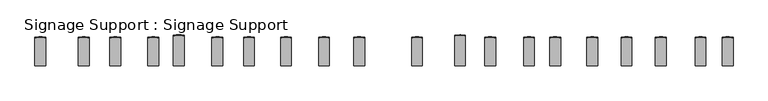
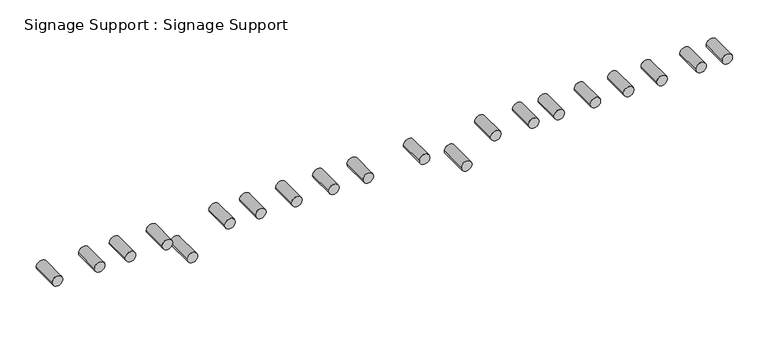
"""IFC4 building model written with IfcOpenShell, lengths in millimetres: proxy geometry, Signage Support : Signage Support."""

import ifcopenshell
import ifcopenshell.guid

model = None  # the IFC model being written
_history = None  # IfcOwnerHistory: only IFC2X3 demands one
_inside = {}  # id of a spatial element -> (the spatial element, [elements in it])
_under = {}  # id of a project, library or spatial element -> (it, [spatial elements below it])
_declared = {}  # id of a project -> (the project, [libraries it declares])
_typed = {}  # id of a type object -> (the type object, [elements of that type])
_made_of = {}  # id of a material, layer set ... -> (it, [elements and type objects made of it])


def new_model(schema):
    """Start an empty IFC model of exactly this schema.

    Asked for "IFC4X3", IfcOpenShell would pick the latest addendum, in which some entities
    have other attributes; the version numbers below select the first issue.
    IFC2X3 requires an IfcOwnerHistory on every rooted entity: one is made here for all.
    """
    global model, _history
    if schema == "IFC4X3":
        model = ifcopenshell.file(schema_version=(4, 3, 0, 0))
    else:
        model = ifcopenshell.file(schema=schema)
    _inside.clear()
    _under.clear()
    _declared.clear()
    _typed.clear()
    _made_of.clear()
    _history = None
    if model.schema == "IFC2X3":
        org = make("IfcOrganization", Name="unknown")
        user = make(
            "IfcPersonAndOrganization",
            ThePerson=make("IfcPerson", FamilyName="unknown"),
            TheOrganization=org,
        )
        app = make(
            "IfcApplication",
            ApplicationDeveloper=org,
            Version="unknown",
            ApplicationFullName="unknown",
            ApplicationIdentifier="unknown",
        )
        _history = make(
            "IfcOwnerHistory",
            OwningUser=user,
            OwningApplication=app,
            ChangeAction="ADDED",
            CreationDate=0,
        )
    return model


def make(cls, **values):
    """One entity of the class cls with the attributes given. An attribute that is None is left unset."""
    return model.create_entity(
        cls, **{name: value for name, value in values.items() if value is not None}
    )


def rooted(cls, **values):
    """An entity with a GlobalId (a new one), such as an element, a storey or a relation."""
    return make(cls, GlobalId=ifcopenshell.guid.new(), OwnerHistory=_history, **values)


def si_unit(unit_type, name, prefix=None):
    """IfcSIUnit, for example si_unit("LENGTHUNIT", "METRE", prefix="MILLI")."""
    return make("IfcSIUnit", UnitType=unit_type, Prefix=prefix, Name=name)


def assignment(units):
    """IfcUnitAssignment: the units of a project."""
    return None if units is None else make("IfcUnitAssignment", Units=units)


def point(xyz):
    """IfcCartesianPoint."""
    return None if xyz is None else make("IfcCartesianPoint", Coordinates=xyz)


def direction(xyz):
    """IfcDirection."""
    return None if xyz is None else make("IfcDirection", DirectionRatios=xyz)


def frame(location, z_axis=None, x_axis=None):
    """IfcAxis2Placement3D, a coordinate frame: its origin and axes. An axis left out is left unset."""
    return make(
        "IfcAxis2Placement3D",
        Location=point(location),
        Axis=direction(z_axis),
        RefDirection=direction(x_axis),
    )


def origin():
    """The frame at (0, 0, 0) with its axes left unset."""
    return frame((0.0, 0.0, 0.0))


def place(relative_to, where):
    """IfcLocalPlacement: puts the frame where relative to a parent placement (None: the world)."""
    return make(
        "IfcLocalPlacement", PlacementRelTo=relative_to, RelativePlacement=where
    )


def context(
    kind, dimensions, precision=None, world=None, true_north=None, identifier=None
):
    """IfcGeometricRepresentationContext, for example the 3D "Model" context."""
    return make(
        "IfcGeometricRepresentationContext",
        ContextIdentifier=identifier,
        ContextType=kind,
        CoordinateSpaceDimension=dimensions,
        Precision=precision,
        WorldCoordinateSystem=world,
        TrueNorth=true_north,
    )


def project(units=None, contexts=None):
    """IfcProject with its units and contexts."""
    return rooted(
        "IfcProject",
        Name="project",
        RepresentationContexts=contexts,
        UnitsInContext=assignment(units),
    )


def spatial(cls, under=None, at=None, **own):
    """A site, building, storey or space (cls), placed at a placement, below another one or the project."""
    s = rooted(cls, ObjectPlacement=at, **own)
    if under is not None:
        _under.setdefault(under.id(), (under, []))[1].append(s)
    return s


def circle_curve(where, radius):
    """IfcCircle in the frame where."""
    return make("IfcCircle", Position=where, Radius=radius)


def ellipse_curve(where, semi_axis1, semi_axis2):
    """IfcEllipse in the frame where."""
    return make(
        "IfcEllipse", Position=where, SemiAxis1=semi_axis1, SemiAxis2=semi_axis2
    )


def shape(context_of_items, identifier, shape_type, items):
    """IfcShapeRepresentation: the items that make up one representation, for example the "Body"."""
    return make(
        "IfcShapeRepresentation",
        ContextOfItems=context_of_items,
        RepresentationIdentifier=identifier,
        RepresentationType=shape_type,
        Items=items,
    )


def source(mapping_origin, context_of_items, identifier, shape_type, items):
    """IfcRepresentationMap: a shape defined once, which mapped items show again and again."""
    return make(
        "IfcRepresentationMap",
        MappingOrigin=mapping_origin,
        MappedRepresentation=shape(context_of_items, identifier, shape_type, items),
    )


def transform(
    local_origin,
    x_axis=None,
    y_axis=None,
    z_axis=None,
    scale=None,
    scale2=None,
    scale3=None,
    uniform=True,
):
    """IfcCartesianTransformationOperator3D, or its non-uniform kind. x_axis, y_axis, z_axis: its Axis1, 2, 3."""
    if uniform:
        return make(
            "IfcCartesianTransformationOperator3D",
            Axis1=direction(x_axis),
            Axis2=direction(y_axis),
            LocalOrigin=point(local_origin),
            Scale=scale,
            Axis3=direction(z_axis),
        )
    return make(
        "IfcCartesianTransformationOperator3DnonUniform",
        Axis1=direction(x_axis),
        Axis2=direction(y_axis),
        LocalOrigin=point(local_origin),
        Scale=scale,
        Axis3=direction(z_axis),
        Scale2=scale2,
        Scale3=scale3,
    )


def mapped(mapping_source, mapping_target):
    """IfcMappedItem: shows the shape of a source again, moved by a transform."""
    return make(
        "IfcMappedItem", MappingSource=mapping_source, MappingTarget=mapping_target
    )


def made_of(thing, what):
    """Note that an element or type object is made of a material, layer set ...; save() writes the relation."""
    if what is not None:
        _made_of.setdefault(what.id(), (what, []))[1].append(thing)
    return thing


def element(
    cls,
    number,
    at=None,
    inside=None,
    cuts=None,
    type_object=None,
    material=None,
    context=None,
    identifier="Body",
    shape_type=None,
    held_by="IfcProductDefinitionShape",
    body=None,
    shapes=None,
    **own,
):
    """One element of the class cls, such as IfcWall. Its Tag is "e" and its number.

    at: its placement. inside: the storey or other place that contains it. cuts: it is an
    opening in that element (IfcRelVoidsElement). A single representation is given by context,
    identifier, shape_type and body (its items); several are given by shapes. held_by: the class
    of the entity that holds the representations. save() writes the other relations.
    """
    e = rooted(cls, Tag="e%d" % number, ObjectPlacement=at, **own)
    if body is not None:
        shapes = [shape(context, identifier, shape_type, body)]
    if shapes is not None:
        e.Representation = make(held_by, Representations=shapes)
    if inside is not None:
        _inside.setdefault(inside.id(), (inside, []))[1].append(e)
    if cuts is not None:
        rooted(
            "IfcRelVoidsElement", RelatingBuildingElement=cuts, RelatedOpeningElement=e
        )
    if type_object is not None:
        _typed.setdefault(type_object.id(), (type_object, []))[1].append(e)
    return made_of(e, material)


def aggregate(whole, parts):
    """IfcRelAggregates: a whole, such as a stair, and the parts it consists of."""
    return rooted("IfcRelAggregates", RelatingObject=whole, RelatedObjects=parts)


def save(model, path):
    """Write the relations noted so far, then the file.

    IfcRelAggregates (storeys below a building ...), IfcRelContainedInSpatialStructure (elements
    in a storey), IfcRelDefinesByType, IfcRelAssociatesMaterial and IfcRelDeclares: one each for
    every whole, place, type object, material and project.
    """
    for whole, parts in _under.values():
        aggregate(whole, parts)
    for where, things in _inside.values():
        rooted(
            "IfcRelContainedInSpatialStructure",
            RelatedElements=things,
            RelatingStructure=where,
        )
    for kind, things in _typed.values():
        rooted("IfcRelDefinesByType", RelatedObjects=things, RelatingType=kind)
    for what, things in _made_of.values():
        rooted("IfcRelAssociatesMaterial", RelatedObjects=things, RelatingMaterial=what)
    for by, libraries in _declared.values():
        rooted("IfcRelDeclares", RelatingContext=by, RelatedDefinitions=libraries)
    model.write(path)


def plane_surface(at):
    """IfcPlane: the flat surface through the origin of the frame at, square to its z axis."""
    return make("IfcPlane", Position=at)


def cylinder_surface(at, radius):
    """IfcCylindricalSurface: all points at the distance radius from the z axis of the frame at."""
    return make("IfcCylindricalSurface", Position=at, Radius=radius)


def advanced_brep(points, edges, surfaces, faces):
    """IfcAdvancedBrep: a solid bounded by faces that lie on surfaces and meet in shared edges.

    An edge is (start, end): straight between two places in points (the first is 0);
    or (start, end, curve); or (start, end, curve, False) where it runs against its curve.
    A face is (place in surfaces, loops), or (place, loops, False) where it looks against
    its surface's normal. A loop lists edges by number (the first is 1), with a minus sign
    where the edge is run from its end to its start. The first loop is the outer one.
    """
    corners = [point(p) for p in points]
    vertices = [make("IfcVertexPoint", VertexGeometry=c) for c in corners]
    made = []
    for start, end, *more in edges:
        made.append(
            make(
                "IfcEdgeCurve",
                EdgeStart=vertices[start],
                EdgeEnd=vertices[end],
                EdgeGeometry=more[0] if more else make("IfcPolyline", Points=[corners[start], corners[end]]),
                SameSense=more[1] if len(more) > 1 else True,
            )
        )
    hull = []
    for where, loops, *sense in faces:
        bounds = []
        for j, loop in enumerate(loops):
            ring = [make("IfcOrientedEdge", EdgeElement=made[abs(k) - 1], Orientation=k > 0) for k in loop]
            bounds.append(
                make(
                    "IfcFaceOuterBound" if j == 0 else "IfcFaceBound",
                    Bound=make("IfcEdgeLoop", EdgeList=ring),
                    Orientation=True,
                )
            )
        hull.append(make("IfcAdvancedFace", Bounds=bounds, FaceSurface=surfaces[where], SameSense=sense[0] if sense else True))
    return make("IfcAdvancedBrep", Outer=make("IfcClosedShell", CfsFaces=hull))


def signage_support_signage_support_2350426c(model_context):
    return source(origin(), model_context, "Body", "AdvancedBrep", [
        advanced_brep(
        [(16177.267357, -19458.5804995, 34584.5182697), (16253.467357, -19458.5804995, 34584.5182697), (16253.467357, -19245.9211169, 34584.5182697), (16177.267357, -19245.9211169, 34584.5182697)],
        [
            (0, 1, circle_curve(frame((16215.367357, -19458.5804995, 34584.5182697), z_axis=(0.0, -1.0, 0.0), x_axis=(1.0, 0.0, 0.0)), 38.1)),
            (1, 0, circle_curve(frame((16215.367357, -19458.5804995, 34584.5182697), z_axis=(0.0, -1.0, 0.0), x_axis=(1.0, 0.0, 0.0)), 38.1)),
            (1, 2),
            (2, 3, ellipse_curve(frame((16215.367357, -19245.9211169, 34584.5182697), z_axis=(0.0, -0.9961946980917453, -0.08715574274766139), x_axis=(0.0, 0.08715574274765964, -0.9961946980917453)), 38.2455358, 38.1)),
            (3, 0),
            (3, 2, ellipse_curve(frame((16215.367357, -19245.9211169, 34584.5182697), z_axis=(0.0, -0.9961946980917453, -0.08715574274766139), x_axis=(0.0, 0.08715574274765964, -0.9961946980917453)), 38.2455358, 38.1)),
        ],
        [
            plane_surface(frame((15807.4961456, -19458.5804995, 34748.2945741), z_axis=(0.0, -1.0, 0.0), x_axis=(0.0, 0.0, 1.0))),
            cylinder_surface(frame((16215.367357, -19458.5804995, 34584.5182697), z_axis=(0.0, 1.0, 0.0), x_axis=(1.0, 0.0, 0.0)), 38.1),
            plane_surface(frame((2527.7462086, -19227.8856773, 34378.3722523), z_axis=(0.0, 0.9961946980917453, 0.08715574274766139), x_axis=(1.0, 0.0, 0.0))),
        ],
        [
            (0, [[1, 2]]),
            (1, [[-2, 3, 4, 5]]),
            (1, [[-1, -5, 6, -3]]),
            (2, [[-4, -6]]),
        ],
    ),
        advanced_brep(
        [(15731.2961456, -19458.5804995, 34748.2945741), (15807.4961456, -19458.5804995, 34748.2945741), (15807.4961456, -19260.2496869, 34748.2945741), (15731.2961456, -19260.2496869, 34748.2945741)],
        [
            (0, 1, circle_curve(frame((15769.3961456, -19458.5804995, 34748.2945741), z_axis=(0.0, 1.0, 0.0), x_axis=(1.0, 0.0, 0.0)), 38.1)),
            (1, 2),
            (2, 3, ellipse_curve(frame((15769.3961456, -19260.2496869, 34748.2945741), z_axis=(0.0, -0.9961946980917453, -0.08715574274766139), x_axis=(0.0, 0.08715574274765964, -0.9961946980917453)), 38.2455358, 38.1)),
            (3, 0),
            (1, 0, circle_curve(frame((15769.3961456, -19458.5804995, 34748.2945741), z_axis=(0.0, 1.0, 0.0), x_axis=(1.0, 0.0, 0.0)), 38.1)),
            (3, 2, ellipse_curve(frame((15769.3961456, -19260.2496869, 34748.2945741), z_axis=(0.0, -0.9961946980917453, -0.08715574274766139), x_axis=(0.0, 0.08715574274765964, -0.9961946980917453)), 38.2455358, 38.1)),
        ],
        [
            cylinder_surface(frame((15769.3961456, -19458.5804995, 34748.2945741), z_axis=(0.0, 1.0, 0.0), x_axis=(1.0, 0.0, 0.0)), 38.1),
            plane_surface(frame((15807.4961456, -19458.5804995, 34748.2945741), z_axis=(0.0, -1.0, 0.0), x_axis=(0.0, 0.0, 1.0))),
            plane_surface(frame((2527.7462086, -19227.8856773, 34378.3722523), z_axis=(0.0, 0.9961946980917453, 0.08715574274766139), x_axis=(1.0, 0.0, 0.0))),
        ],
        [
            (0, [[1, 2, 3, 4]]),
            (0, [[5, -4, 6, -2]]),
            (1, [[-5, -1]]),
            (2, [[-3, -6]]),
        ],
    ),
        advanced_brep(
        [(15997.9961456, -19458.5804995, 34748.2945741), (16074.1961456, -19458.5804995, 34748.2945741), (16074.1961456, -19260.2496869, 34748.2945741), (15997.9961456, -19260.2496869, 34748.2945741)],
        [
            (0, 1, circle_curve(frame((16036.0961456, -19458.5804995, 34748.2945741), z_axis=(0.0, 1.0, 0.0), x_axis=(1.0, 0.0, 0.0)), 38.1)),
            (1, 2),
            (2, 3, ellipse_curve(frame((16036.0961456, -19260.2496869, 34748.2945741), z_axis=(0.0, -0.9961946980917453, -0.08715574274766139), x_axis=(0.0, 0.08715574274765964, -0.9961946980917453)), 38.2455358, 38.1)),
            (3, 0),
            (1, 0, circle_curve(frame((16036.0961456, -19458.5804995, 34748.2945741), z_axis=(0.0, 1.0, 0.0), x_axis=(1.0, 0.0, 0.0)), 38.1)),
            (3, 2, ellipse_curve(frame((16036.0961456, -19260.2496869, 34748.2945741), z_axis=(0.0, -0.9961946980917453, -0.08715574274766139), x_axis=(0.0, 0.08715574274765964, -0.9961946980917453)), 38.2455358, 38.1)),
        ],
        [
            cylinder_surface(frame((16036.0961456, -19458.5804995, 34748.2945741), z_axis=(0.0, 1.0, 0.0), x_axis=(1.0, 0.0, 0.0)), 38.1),
            plane_surface(frame((15807.4961456, -19458.5804995, 34748.2945741), z_axis=(0.0, -1.0, 0.0), x_axis=(0.0, 0.0, 1.0))),
            plane_surface(frame((2527.7462086, -19227.8856773, 34378.3722523), z_axis=(0.0, 0.9961946980917453, 0.08715574274766139), x_axis=(1.0, 0.0, 0.0))),
        ],
        [
            (0, [[1, 2, 3, 4]]),
            (0, [[5, -4, 6, -2]]),
            (1, [[-5, -1]]),
            (2, [[-3, -6]]),
        ],
    ),
        advanced_brep(
        [(16448.8461456, -19458.5804995, 34748.2945741), (16525.0461456, -19458.5804995, 34748.2945741), (16525.0461456, -19260.2496869, 34748.2945741), (16448.8461456, -19260.2496869, 34748.2945741)],
        [
            (0, 1, circle_curve(frame((16486.9461456, -19458.5804995, 34748.2945741), z_axis=(0.0, 1.0, 0.0), x_axis=(1.0, 0.0, 0.0)), 38.1)),
            (1, 2),
            (2, 3, ellipse_curve(frame((16486.9461456, -19260.2496869, 34748.2945741), z_axis=(0.0, -0.9961946980917453, -0.08715574274766139), x_axis=(0.0, 0.08715574274765964, -0.9961946980917453)), 38.2455358, 38.1)),
            (3, 0),
            (1, 0, circle_curve(frame((16486.9461456, -19458.5804995, 34748.2945741), z_axis=(0.0, 1.0, 0.0), x_axis=(1.0, 0.0, 0.0)), 38.1)),
            (3, 2, ellipse_curve(frame((16486.9461456, -19260.2496869, 34748.2945741), z_axis=(0.0, -0.9961946980917453, -0.08715574274766139), x_axis=(0.0, 0.08715574274765964, -0.9961946980917453)), 38.2455358, 38.1)),
        ],
        [
            cylinder_surface(frame((16486.9461456, -19458.5804995, 34748.2945741), z_axis=(0.0, 1.0, 0.0), x_axis=(1.0, 0.0, 0.0)), 38.1),
            plane_surface(frame((15807.4961456, -19458.5804995, 34748.2945741), z_axis=(0.0, -1.0, 0.0), x_axis=(0.0, 0.0, 1.0))),
            plane_surface(frame((2527.7462086, -19227.8856773, 34378.3722523), z_axis=(0.0, 0.9961946980917453, 0.08715574274766139), x_axis=(1.0, 0.0, 0.0))),
        ],
        [
            (0, [[1, 2, 3, 4]]),
            (0, [[5, -4, 6, -2]]),
            (1, [[-5, -1]]),
            (2, [[-3, -6]]),
        ],
    ),
        advanced_brep(
        [(15509.0461456, -19458.5804995, 34748.2945741), (15585.2461456, -19458.5804995, 34748.2945741), (15585.2461456, -19260.2496869, 34748.2945741), (15509.0461456, -19260.2496869, 34748.2945741)],
        [
            (0, 1, circle_curve(frame((15547.1461456, -19458.5804995, 34748.2945741), z_axis=(0.0, 1.0, 0.0), x_axis=(1.0, 0.0, 0.0)), 38.1)),
            (1, 2),
            (2, 3, ellipse_curve(frame((15547.1461456, -19260.2496869, 34748.2945741), z_axis=(0.0, -0.9961946980917453, -0.08715574274766139), x_axis=(0.0, 0.08715574274765964, -0.9961946980917453)), 38.2455358, 38.1)),
            (3, 0),
            (1, 0, circle_curve(frame((15547.1461456, -19458.5804995, 34748.2945741), z_axis=(0.0, 1.0, 0.0), x_axis=(1.0, 0.0, 0.0)), 38.1)),
            (3, 2, ellipse_curve(frame((15547.1461456, -19260.2496869, 34748.2945741), z_axis=(0.0, -0.9961946980917453, -0.08715574274766139), x_axis=(0.0, 0.08715574274765964, -0.9961946980917453)), 38.2455358, 38.1)),
        ],
        [
            cylinder_surface(frame((15547.1461456, -19458.5804995, 34748.2945741), z_axis=(0.0, 1.0, 0.0), x_axis=(1.0, 0.0, 0.0)), 38.1),
            plane_surface(frame((15807.4961456, -19458.5804995, 34748.2945741), z_axis=(0.0, -1.0, 0.0), x_axis=(0.0, 0.0, 1.0))),
            plane_surface(frame((2527.7462086, -19227.8856773, 34378.3722523), z_axis=(0.0, 0.9961946980917453, 0.08715574274766139), x_axis=(1.0, 0.0, 0.0))),
        ],
        [
            (0, [[1, 2, 3, 4]]),
            (0, [[5, -4, 6, -2]]),
            (1, [[-5, -1]]),
            (2, [[-3, -6]]),
        ],
    ),
        advanced_brep(
        [(15204.2461456, -19458.5804995, 34748.2945741), (15280.4461456, -19458.5804995, 34748.2945741), (15280.4461456, -19260.2496869, 34748.2945741), (15204.2461456, -19260.2496869, 34748.2945741)],
        [
            (0, 1, circle_curve(frame((15242.3461456, -19458.5804995, 34748.2945741), z_axis=(0.0, 1.0, 0.0), x_axis=(1.0, 0.0, 0.0)), 38.1)),
            (1, 2),
            (2, 3, ellipse_curve(frame((15242.3461456, -19260.2496869, 34748.2945741), z_axis=(0.0, -0.9961946980917453, -0.08715574274766139), x_axis=(0.0, 0.08715574274765964, -0.9961946980917453)), 38.2455358, 38.1)),
            (3, 0),
            (1, 0, circle_curve(frame((15242.3461456, -19458.5804995, 34748.2945741), z_axis=(0.0, 1.0, 0.0), x_axis=(1.0, 0.0, 0.0)), 38.1)),
            (3, 2, ellipse_curve(frame((15242.3461456, -19260.2496869, 34748.2945741), z_axis=(0.0, -0.9961946980917453, -0.08715574274766139), x_axis=(0.0, 0.08715574274765964, -0.9961946980917453)), 38.2455358, 38.1)),
        ],
        [
            cylinder_surface(frame((15242.3461456, -19458.5804995, 34748.2945741), z_axis=(0.0, 1.0, 0.0), x_axis=(1.0, 0.0, 0.0)), 38.1),
            plane_surface(frame((15807.4961456, -19458.5804995, 34748.2945741), z_axis=(0.0, -1.0, 0.0), x_axis=(0.0, 0.0, 1.0))),
            plane_surface(frame((2527.7462086, -19227.8856773, 34378.3722523), z_axis=(0.0, 0.9961946980917453, 0.08715574274766139), x_axis=(1.0, 0.0, 0.0))),
        ],
        [
            (0, [[1, 2, 3, 4]]),
            (0, [[5, -4, 6, -2]]),
            (1, [[-5, -1]]),
            (2, [[-3, -6]]),
        ],
    ),
        advanced_brep(
        [(16671.0961456, -19458.5804995, 34748.2945741), (16747.2961456, -19458.5804995, 34748.2945741), (16747.2961456, -19260.2496869, 34748.2945741), (16671.0961456, -19260.2496869, 34748.2945741)],
        [
            (0, 1, circle_curve(frame((16709.1961456, -19458.5804995, 34748.2945741), z_axis=(0.0, 1.0, 0.0), x_axis=(1.0, 0.0, 0.0)), 38.1)),
            (1, 2),
            (2, 3, ellipse_curve(frame((16709.1961456, -19260.2496869, 34748.2945741), z_axis=(0.0, -0.9961946980917453, -0.08715574274766139), x_axis=(0.0, 0.08715574274765964, -0.9961946980917453)), 38.2455358, 38.1)),
            (3, 0),
            (1, 0, circle_curve(frame((16709.1961456, -19458.5804995, 34748.2945741), z_axis=(0.0, 1.0, 0.0), x_axis=(1.0, 0.0, 0.0)), 38.1)),
            (3, 2, ellipse_curve(frame((16709.1961456, -19260.2496869, 34748.2945741), z_axis=(0.0, -0.9961946980917453, -0.08715574274766139), x_axis=(0.0, 0.08715574274765964, -0.9961946980917453)), 38.2455358, 38.1)),
        ],
        [
            cylinder_surface(frame((16709.1961456, -19458.5804995, 34748.2945741), z_axis=(0.0, 1.0, 0.0), x_axis=(1.0, 0.0, 0.0)), 38.1),
            plane_surface(frame((15807.4961456, -19458.5804995, 34748.2945741), z_axis=(0.0, -1.0, 0.0), x_axis=(0.0, 0.0, 1.0))),
            plane_surface(frame((2527.7462086, -19227.8856773, 34378.3722523), z_axis=(0.0, 0.9961946980917453, 0.08715574274766139), x_axis=(1.0, 0.0, 0.0))),
        ],
        [
            (0, [[1, 2, 3, 4]]),
            (0, [[5, -4, 6, -2]]),
            (1, [[-5, -1]]),
            (2, [[-3, -6]]),
        ],
    ),
        advanced_brep(
        [(16931.4461456, -19458.5804995, 34748.2945741), (17007.6461456, -19458.5804995, 34748.2945741), (17007.6461456, -19260.2496869, 34748.2945741), (16931.4461456, -19260.2496869, 34748.2945741)],
        [
            (0, 1, circle_curve(frame((16969.5461456, -19458.5804995, 34748.2945741), z_axis=(0.0, 1.0, 0.0), x_axis=(1.0, 0.0, 0.0)), 38.1)),
            (1, 2),
            (2, 3, ellipse_curve(frame((16969.5461456, -19260.2496869, 34748.2945741), z_axis=(0.0, -0.9961946980917453, -0.08715574274766139), x_axis=(0.0, 0.08715574274765964, -0.9961946980917453)), 38.2455358, 38.1)),
            (3, 0),
            (1, 0, circle_curve(frame((16969.5461456, -19458.5804995, 34748.2945741), z_axis=(0.0, 1.0, 0.0), x_axis=(1.0, 0.0, 0.0)), 38.1)),
            (3, 2, ellipse_curve(frame((16969.5461456, -19260.2496869, 34748.2945741), z_axis=(0.0, -0.9961946980917453, -0.08715574274766139), x_axis=(0.0, 0.08715574274765964, -0.9961946980917453)), 38.2455358, 38.1)),
        ],
        [
            cylinder_surface(frame((16969.5461456, -19458.5804995, 34748.2945741), z_axis=(0.0, 1.0, 0.0), x_axis=(1.0, 0.0, 0.0)), 38.1),
            plane_surface(frame((15807.4961456, -19458.5804995, 34748.2945741), z_axis=(0.0, -1.0, 0.0), x_axis=(0.0, 0.0, 1.0))),
            plane_surface(frame((2527.7462086, -19227.8856773, 34378.3722523), z_axis=(0.0, 0.9961946980917453, 0.08715574274766139), x_axis=(1.0, 0.0, 0.0))),
        ],
        [
            (0, [[1, 2, 3, 4]]),
            (0, [[5, -4, 6, -2]]),
            (1, [[-5, -1]]),
            (2, [[-3, -6]]),
        ],
    ),
        advanced_brep(
        [(17198.1461456, -19458.5804995, 34748.2945741), (17274.3461456, -19458.5804995, 34748.2945741), (17274.3461456, -19260.2496869, 34748.2945741), (17198.1461456, -19260.2496869, 34748.2945741)],
        [
            (0, 1, circle_curve(frame((17236.2461456, -19458.5804995, 34748.2945741), z_axis=(0.0, 1.0, 0.0), x_axis=(1.0, 0.0, 0.0)), 38.1)),
            (1, 2),
            (2, 3, ellipse_curve(frame((17236.2461456, -19260.2496869, 34748.2945741), z_axis=(0.0, -0.9961946980917453, -0.08715574274766139), x_axis=(0.0, 0.08715574274765964, -0.9961946980917453)), 38.2455358, 38.1)),
            (3, 0),
            (1, 0, circle_curve(frame((17236.2461456, -19458.5804995, 34748.2945741), z_axis=(0.0, 1.0, 0.0), x_axis=(1.0, 0.0, 0.0)), 38.1)),
            (3, 2, ellipse_curve(frame((17236.2461456, -19260.2496869, 34748.2945741), z_axis=(0.0, -0.9961946980917453, -0.08715574274766139), x_axis=(0.0, 0.08715574274765964, -0.9961946980917453)), 38.2455358, 38.1)),
        ],
        [
            cylinder_surface(frame((17236.2461456, -19458.5804995, 34748.2945741), z_axis=(0.0, 1.0, 0.0), x_axis=(1.0, 0.0, 0.0)), 38.1),
            plane_surface(frame((15807.4961456, -19458.5804995, 34748.2945741), z_axis=(0.0, -1.0, 0.0), x_axis=(0.0, 0.0, 1.0))),
            plane_surface(frame((2527.7462086, -19227.8856773, 34378.3722523), z_axis=(0.0, 0.9961946980917453, 0.08715574274766139), x_axis=(1.0, 0.0, 0.0))),
        ],
        [
            (0, [[1, 2, 3, 4]]),
            (0, [[5, -4, 6, -2]]),
            (1, [[-5, -1]]),
            (2, [[-3, -6]]),
        ],
    ),
        advanced_brep(
        [(17445.7961456, -19458.5804995, 34748.2945741), (17521.9961456, -19458.5804995, 34748.2945741), (17521.9961456, -19260.2496869, 34748.2945741), (17445.7961456, -19260.2496869, 34748.2945741)],
        [
            (0, 1, circle_curve(frame((17483.8961456, -19458.5804995, 34748.2945741), z_axis=(0.0, 1.0, 0.0), x_axis=(1.0, 0.0, 0.0)), 38.1)),
            (1, 2),
            (2, 3, ellipse_curve(frame((17483.8961456, -19260.2496869, 34748.2945741), z_axis=(0.0, -0.9961946980917453, -0.08715574274766139), x_axis=(0.0, 0.08715574274765964, -0.9961946980917453)), 38.2455358, 38.1)),
            (3, 0),
            (1, 0, circle_curve(frame((17483.8961456, -19458.5804995, 34748.2945741), z_axis=(0.0, 1.0, 0.0), x_axis=(1.0, 0.0, 0.0)), 38.1)),
            (3, 2, ellipse_curve(frame((17483.8961456, -19260.2496869, 34748.2945741), z_axis=(0.0, -0.9961946980917453, -0.08715574274766139), x_axis=(0.0, 0.08715574274765964, -0.9961946980917453)), 38.2455358, 38.1)),
        ],
        [
            cylinder_surface(frame((17483.8961456, -19458.5804995, 34748.2945741), z_axis=(0.0, 1.0, 0.0), x_axis=(1.0, 0.0, 0.0)), 38.1),
            plane_surface(frame((15807.4961456, -19458.5804995, 34748.2945741), z_axis=(0.0, -1.0, 0.0), x_axis=(0.0, 0.0, 1.0))),
            plane_surface(frame((2527.7462086, -19227.8856773, 34378.3722523), z_axis=(0.0, 0.9961946980917453, 0.08715574274766139), x_axis=(1.0, 0.0, 0.0))),
        ],
        [
            (0, [[1, 2, 3, 4]]),
            (0, [[5, -4, 6, -2]]),
            (1, [[-5, -1]]),
            (2, [[-3, -6]]),
        ],
    ),
        advanced_brep(
        [(17852.1961456, -19458.5804995, 34748.2945741), (17928.3961456, -19458.5804995, 34748.2945741), (17928.3961456, -19260.2496869, 34748.2945741), (17852.1961456, -19260.2496869, 34748.2945741)],
        [
            (0, 1, circle_curve(frame((17890.2961456, -19458.5804995, 34748.2945741), z_axis=(0.0, 1.0, 0.0), x_axis=(1.0, 0.0, 0.0)), 38.1)),
            (1, 2),
            (2, 3, ellipse_curve(frame((17890.2961456, -19260.2496869, 34748.2945741), z_axis=(0.0, -0.9961946980917453, -0.08715574274766139), x_axis=(0.0, 0.08715574274765964, -0.9961946980917453)), 38.2455358, 38.1)),
            (3, 0),
            (1, 0, circle_curve(frame((17890.2961456, -19458.5804995, 34748.2945741), z_axis=(0.0, 1.0, 0.0), x_axis=(1.0, 0.0, 0.0)), 38.1)),
            (3, 2, ellipse_curve(frame((17890.2961456, -19260.2496869, 34748.2945741), z_axis=(0.0, -0.9961946980917453, -0.08715574274766139), x_axis=(0.0, 0.08715574274765964, -0.9961946980917453)), 38.2455358, 38.1)),
        ],
        [
            cylinder_surface(frame((17890.2961456, -19458.5804995, 34748.2945741), z_axis=(0.0, 1.0, 0.0), x_axis=(1.0, 0.0, 0.0)), 38.1),
            plane_surface(frame((15807.4961456, -19458.5804995, 34748.2945741), z_axis=(0.0, -1.0, 0.0), x_axis=(0.0, 0.0, 1.0))),
            plane_surface(frame((2527.7462086, -19227.8856773, 34378.3722523), z_axis=(0.0, 0.9961946980917453, 0.08715574274766139), x_axis=(1.0, 0.0, 0.0))),
        ],
        [
            (0, [[1, 2, 3, 4]]),
            (0, [[5, -4, 6, -2]]),
            (1, [[-5, -1]]),
            (2, [[-3, -6]]),
        ],
    ),
        advanced_brep(
        [(18366.5461456, -19458.5804995, 34748.2945741), (18442.7461456, -19458.5804995, 34748.2945741), (18442.7461456, -19260.2496869, 34748.2945741), (18366.5461456, -19260.2496869, 34748.2945741)],
        [
            (0, 1, circle_curve(frame((18404.6461456, -19458.5804995, 34748.2945741), z_axis=(0.0, 1.0, 0.0), x_axis=(1.0, 0.0, 0.0)), 38.1)),
            (1, 2),
            (2, 3, ellipse_curve(frame((18404.6461456, -19260.2496869, 34748.2945741), z_axis=(0.0, -0.9961946980917453, -0.08715574274766139), x_axis=(0.0, 0.08715574274765964, -0.9961946980917453)), 38.2455358, 38.1)),
            (3, 0),
            (1, 0, circle_curve(frame((18404.6461456, -19458.5804995, 34748.2945741), z_axis=(0.0, 1.0, 0.0), x_axis=(1.0, 0.0, 0.0)), 38.1)),
            (3, 2, ellipse_curve(frame((18404.6461456, -19260.2496869, 34748.2945741), z_axis=(0.0, -0.9961946980917453, -0.08715574274766139), x_axis=(0.0, 0.08715574274765964, -0.9961946980917453)), 38.2455358, 38.1)),
        ],
        [
            cylinder_surface(frame((18404.6461456, -19458.5804995, 34748.2945741), z_axis=(0.0, 1.0, 0.0), x_axis=(1.0, 0.0, 0.0)), 38.1),
            plane_surface(frame((15807.4961456, -19458.5804995, 34748.2945741), z_axis=(0.0, -1.0, 0.0), x_axis=(0.0, 0.0, 1.0))),
            plane_surface(frame((2527.7462086, -19227.8856773, 34378.3722523), z_axis=(0.0, 0.9961946980917453, 0.08715574274766139), x_axis=(1.0, 0.0, 0.0))),
        ],
        [
            (0, [[1, 2, 3, 4]]),
            (0, [[5, -4, 6, -2]]),
            (1, [[-5, -1]]),
            (2, [[-3, -6]]),
        ],
    ),
        advanced_brep(
        [(18639.5961456, -19458.5804995, 34748.2945741), (18715.7961456, -19458.5804995, 34748.2945741), (18715.7961456, -19260.2496869, 34748.2945741), (18639.5961456, -19260.2496869, 34748.2945741)],
        [
            (0, 1, circle_curve(frame((18677.6961456, -19458.5804995, 34748.2945741), z_axis=(0.0, 1.0, 0.0), x_axis=(1.0, 0.0, 0.0)), 38.1)),
            (1, 2),
            (2, 3, ellipse_curve(frame((18677.6961456, -19260.2496869, 34748.2945741), z_axis=(0.0, -0.9961946980917453, -0.08715574274766139), x_axis=(0.0, 0.08715574274765964, -0.9961946980917453)), 38.2455358, 38.1)),
            (3, 0),
            (1, 0, circle_curve(frame((18677.6961456, -19458.5804995, 34748.2945741), z_axis=(0.0, 1.0, 0.0), x_axis=(1.0, 0.0, 0.0)), 38.1)),
            (3, 2, ellipse_curve(frame((18677.6961456, -19260.2496869, 34748.2945741), z_axis=(0.0, -0.9961946980917453, -0.08715574274766139), x_axis=(0.0, 0.08715574274765964, -0.9961946980917453)), 38.2455358, 38.1)),
        ],
        [
            cylinder_surface(frame((18677.6961456, -19458.5804995, 34748.2945741), z_axis=(0.0, 1.0, 0.0), x_axis=(1.0, 0.0, 0.0)), 38.1),
            plane_surface(frame((15807.4961456, -19458.5804995, 34748.2945741), z_axis=(0.0, -1.0, 0.0), x_axis=(0.0, 0.0, 1.0))),
            plane_surface(frame((2527.7462086, -19227.8856773, 34378.3722523), z_axis=(0.0, 0.9961946980917453, 0.08715574274766139), x_axis=(1.0, 0.0, 0.0))),
        ],
        [
            (0, [[1, 2, 3, 4]]),
            (0, [[5, -4, 6, -2]]),
            (1, [[-5, -1]]),
            (2, [[-3, -6]]),
        ],
    ),
        advanced_brep(
        [(18823.7461456, -19458.5804995, 34748.2945741), (18899.9461456, -19458.5804995, 34748.2945741), (18899.9461456, -19260.2496869, 34748.2945741), (18823.7461456, -19260.2496869, 34748.2945741)],
        [
            (0, 1, circle_curve(frame((18861.8461456, -19458.5804995, 34748.2945741), z_axis=(0.0, 1.0, 0.0), x_axis=(1.0, 0.0, 0.0)), 38.1)),
            (1, 2),
            (2, 3, ellipse_curve(frame((18861.8461456, -19260.2496869, 34748.2945741), z_axis=(0.0, -0.9961946980917453, -0.08715574274766139), x_axis=(0.0, 0.08715574274765964, -0.9961946980917453)), 38.2455358, 38.1)),
            (3, 0),
            (1, 0, circle_curve(frame((18861.8461456, -19458.5804995, 34748.2945741), z_axis=(0.0, 1.0, 0.0), x_axis=(1.0, 0.0, 0.0)), 38.1)),
            (3, 2, ellipse_curve(frame((18861.8461456, -19260.2496869, 34748.2945741), z_axis=(0.0, -0.9961946980917453, -0.08715574274766139), x_axis=(0.0, 0.08715574274765964, -0.9961946980917453)), 38.2455358, 38.1)),
        ],
        [
            cylinder_surface(frame((18861.8461456, -19458.5804995, 34748.2945741), z_axis=(0.0, 1.0, 0.0), x_axis=(1.0, 0.0, 0.0)), 38.1),
            plane_surface(frame((15807.4961456, -19458.5804995, 34748.2945741), z_axis=(0.0, -1.0, 0.0), x_axis=(0.0, 0.0, 1.0))),
            plane_surface(frame((2527.7462086, -19227.8856773, 34378.3722523), z_axis=(0.0, 0.9961946980917453, 0.08715574274766139), x_axis=(1.0, 0.0, 0.0))),
        ],
        [
            (0, [[1, 2, 3, 4]]),
            (0, [[5, -4, 6, -2]]),
            (1, [[-5, -1]]),
            (2, [[-3, -6]]),
        ],
    ),
        advanced_brep(
        [(19084.0961456, -19458.5804995, 34748.2945741), (19160.2961456, -19458.5804995, 34748.2945741), (19160.2961456, -19260.2496869, 34748.2945741), (19084.0961456, -19260.2496869, 34748.2945741)],
        [
            (0, 1, circle_curve(frame((19122.1961456, -19458.5804995, 34748.2945741), z_axis=(0.0, 1.0, 0.0), x_axis=(1.0, 0.0, 0.0)), 38.1)),
            (1, 2),
            (2, 3, ellipse_curve(frame((19122.1961456, -19260.2496869, 34748.2945741), z_axis=(0.0, -0.9961946980917453, -0.08715574274766139), x_axis=(0.0, 0.08715574274765964, -0.9961946980917453)), 38.2455358, 38.1)),
            (3, 0),
            (1, 0, circle_curve(frame((19122.1961456, -19458.5804995, 34748.2945741), z_axis=(0.0, 1.0, 0.0), x_axis=(1.0, 0.0, 0.0)), 38.1)),
            (3, 2, ellipse_curve(frame((19122.1961456, -19260.2496869, 34748.2945741), z_axis=(0.0, -0.9961946980917453, -0.08715574274766139), x_axis=(0.0, 0.08715574274765964, -0.9961946980917453)), 38.2455358, 38.1)),
        ],
        [
            cylinder_surface(frame((19122.1961456, -19458.5804995, 34748.2945741), z_axis=(0.0, 1.0, 0.0), x_axis=(1.0, 0.0, 0.0)), 38.1),
            plane_surface(frame((15807.4961456, -19458.5804995, 34748.2945741), z_axis=(0.0, -1.0, 0.0), x_axis=(0.0, 0.0, 1.0))),
            plane_surface(frame((2527.7462086, -19227.8856773, 34378.3722523), z_axis=(0.0, 0.9961946980917453, 0.08715574274766139), x_axis=(1.0, 0.0, 0.0))),
        ],
        [
            (0, [[1, 2, 3, 4]]),
            (0, [[5, -4, 6, -2]]),
            (1, [[-5, -1]]),
            (2, [[-3, -6]]),
        ],
    ),
        advanced_brep(
        [(19325.3961456, -19458.5804995, 34748.2945741), (19401.5961456, -19458.5804995, 34748.2945741), (19401.5961456, -19260.2496869, 34748.2945741), (19325.3961456, -19260.2496869, 34748.2945741)],
        [
            (0, 1, circle_curve(frame((19363.4961456, -19458.5804995, 34748.2945741), z_axis=(0.0, 1.0, 0.0), x_axis=(1.0, 0.0, 0.0)), 38.1)),
            (1, 2),
            (2, 3, ellipse_curve(frame((19363.4961456, -19260.2496869, 34748.2945741), z_axis=(0.0, -0.9961946980917453, -0.08715574274766139), x_axis=(0.0, 0.08715574274765964, -0.9961946980917453)), 38.2455358, 38.1)),
            (3, 0),
            (1, 0, circle_curve(frame((19363.4961456, -19458.5804995, 34748.2945741), z_axis=(0.0, 1.0, 0.0), x_axis=(1.0, 0.0, 0.0)), 38.1)),
            (3, 2, ellipse_curve(frame((19363.4961456, -19260.2496869, 34748.2945741), z_axis=(0.0, -0.9961946980917453, -0.08715574274766139), x_axis=(0.0, 0.08715574274765964, -0.9961946980917453)), 38.2455358, 38.1)),
        ],
        [
            cylinder_surface(frame((19363.4961456, -19458.5804995, 34748.2945741), z_axis=(0.0, 1.0, 0.0), x_axis=(1.0, 0.0, 0.0)), 38.1),
            plane_surface(frame((15807.4961456, -19458.5804995, 34748.2945741), z_axis=(0.0, -1.0, 0.0), x_axis=(0.0, 0.0, 1.0))),
            plane_surface(frame((2527.7462086, -19227.8856773, 34378.3722523), z_axis=(0.0, 0.9961946980917453, 0.08715574274766139), x_axis=(1.0, 0.0, 0.0))),
        ],
        [
            (0, [[1, 2, 3, 4]]),
            (0, [[5, -4, 6, -2]]),
            (1, [[-5, -1]]),
            (2, [[-3, -6]]),
        ],
    ),
        advanced_brep(
        [(19566.6961456, -19458.5804995, 34748.2945741), (19642.8961456, -19458.5804995, 34748.2945741), (19642.8961456, -19260.2496869, 34748.2945741), (19566.6961456, -19260.2496869, 34748.2945741)],
        [
            (0, 1, circle_curve(frame((19604.7961456, -19458.5804995, 34748.2945741), z_axis=(0.0, 1.0, 0.0), x_axis=(1.0, 0.0, 0.0)), 38.1)),
            (1, 2),
            (2, 3, ellipse_curve(frame((19604.7961456, -19260.2496869, 34748.2945741), z_axis=(0.0, -0.9961946980917453, -0.08715574274766139), x_axis=(0.0, 0.08715574274765964, -0.9961946980917453)), 38.2455358, 38.1)),
            (3, 0),
            (1, 0, circle_curve(frame((19604.7961456, -19458.5804995, 34748.2945741), z_axis=(0.0, 1.0, 0.0), x_axis=(1.0, 0.0, 0.0)), 38.1)),
            (3, 2, ellipse_curve(frame((19604.7961456, -19260.2496869, 34748.2945741), z_axis=(0.0, -0.9961946980917453, -0.08715574274766139), x_axis=(0.0, 0.08715574274765964, -0.9961946980917453)), 38.2455358, 38.1)),
        ],
        [
            cylinder_surface(frame((19604.7961456, -19458.5804995, 34748.2945741), z_axis=(0.0, 1.0, 0.0), x_axis=(1.0, 0.0, 0.0)), 38.1),
            plane_surface(frame((15807.4961456, -19458.5804995, 34748.2945741), z_axis=(0.0, -1.0, 0.0), x_axis=(0.0, 0.0, 1.0))),
            plane_surface(frame((2527.7462086, -19227.8856773, 34378.3722523), z_axis=(0.0, 0.9961946980917453, 0.08715574274766139), x_axis=(1.0, 0.0, 0.0))),
        ],
        [
            (0, [[1, 2, 3, 4]]),
            (0, [[5, -4, 6, -2]]),
            (1, [[-5, -1]]),
            (2, [[-3, -6]]),
        ],
    ),
        advanced_brep(
        [(19846.0961456, -19458.5804995, 34748.2945741), (19922.2961456, -19458.5804995, 34748.2945741), (19922.2961456, -19260.2496869, 34748.2945741), (19846.0961456, -19260.2496869, 34748.2945741)],
        [
            (0, 1, circle_curve(frame((19884.1961456, -19458.5804995, 34748.2945741), z_axis=(0.0, 1.0, 0.0), x_axis=(1.0, 0.0, 0.0)), 38.1)),
            (1, 2),
            (2, 3, ellipse_curve(frame((19884.1961456, -19260.2496869, 34748.2945741), z_axis=(0.0, -0.9961946980917453, -0.08715574274766139), x_axis=(0.0, 0.08715574274765964, -0.9961946980917453)), 38.2455358, 38.1)),
            (3, 0),
            (1, 0, circle_curve(frame((19884.1961456, -19458.5804995, 34748.2945741), z_axis=(0.0, 1.0, 0.0), x_axis=(1.0, 0.0, 0.0)), 38.1)),
            (3, 2, ellipse_curve(frame((19884.1961456, -19260.2496869, 34748.2945741), z_axis=(0.0, -0.9961946980917453, -0.08715574274766139), x_axis=(0.0, 0.08715574274765964, -0.9961946980917453)), 38.2455358, 38.1)),
        ],
        [
            cylinder_surface(frame((19884.1961456, -19458.5804995, 34748.2945741), z_axis=(0.0, 1.0, 0.0), x_axis=(1.0, 0.0, 0.0)), 38.1),
            plane_surface(frame((15807.4961456, -19458.5804995, 34748.2945741), z_axis=(0.0, -1.0, 0.0), x_axis=(0.0, 0.0, 1.0))),
            plane_surface(frame((2527.7462086, -19227.8856773, 34378.3722523), z_axis=(0.0, 0.9961946980917453, 0.08715574274766139), x_axis=(1.0, 0.0, 0.0))),
        ],
        [
            (0, [[1, 2, 3, 4]]),
            (0, [[5, -4, 6, -2]]),
            (1, [[-5, -1]]),
            (2, [[-3, -6]]),
        ],
    ),
        advanced_brep(
        [(20036.5961456, -19458.5804995, 34748.2945741), (20112.7961456, -19458.5804995, 34748.2945741), (20112.7961456, -19260.2496869, 34748.2945741), (20036.5961456, -19260.2496869, 34748.2945741)],
        [
            (0, 1, circle_curve(frame((20074.6961456, -19458.5804995, 34748.2945741), z_axis=(0.0, 1.0, 0.0), x_axis=(1.0, 0.0, 0.0)), 38.1)),
            (1, 2),
            (2, 3, ellipse_curve(frame((20074.6961456, -19260.2496869, 34748.2945741), z_axis=(0.0, -0.9961946980917453, -0.08715574274766139), x_axis=(0.0, 0.08715574274765964, -0.9961946980917453)), 38.2455358, 38.1)),
            (3, 0),
            (1, 0, circle_curve(frame((20074.6961456, -19458.5804995, 34748.2945741), z_axis=(0.0, 1.0, 0.0), x_axis=(1.0, 0.0, 0.0)), 38.1)),
            (3, 2, ellipse_curve(frame((20074.6961456, -19260.2496869, 34748.2945741), z_axis=(0.0, -0.9961946980917453, -0.08715574274766139), x_axis=(0.0, 0.08715574274765964, -0.9961946980917453)), 38.2455358, 38.1)),
        ],
        [
            cylinder_surface(frame((20074.6961456, -19458.5804995, 34748.2945741), z_axis=(0.0, 1.0, 0.0), x_axis=(1.0, 0.0, 0.0)), 38.1),
            plane_surface(frame((15807.4961456, -19458.5804995, 34748.2945741), z_axis=(0.0, -1.0, 0.0), x_axis=(0.0, 0.0, 1.0))),
            plane_surface(frame((2527.7462086, -19227.8856773, 34378.3722523), z_axis=(0.0, 0.9961946980917453, 0.08715574274766139), x_axis=(1.0, 0.0, 0.0))),
        ],
        [
            (0, [[1, 2, 3, 4]]),
            (0, [[5, -4, 6, -2]]),
            (1, [[-5, -1]]),
            (2, [[-3, -6]]),
        ],
    ),
        advanced_brep(
        [(18155.240225, -19458.5804995, 34591.3373524), (18231.440225, -19458.5804995, 34591.3373524), (18231.440225, -19246.5177093, 34591.3373524), (18155.240225, -19246.5177093, 34591.3373524)],
        [
            (0, 1, circle_curve(frame((18193.340225, -19458.5804995, 34591.3373524), z_axis=(0.0, 1.0, 0.0), x_axis=(1.0, 0.0, 0.0)), 38.1)),
            (1, 2),
            (2, 3, ellipse_curve(frame((18193.340225, -19246.5177093, 34591.3373524), z_axis=(0.0, -0.9961946980917453, -0.08715574274766139), x_axis=(0.0, 0.08715574274765964, -0.9961946980917453)), 38.2455358, 38.1)),
            (3, 0),
            (1, 0, circle_curve(frame((18193.340225, -19458.5804995, 34591.3373524), z_axis=(0.0, 1.0, 0.0), x_axis=(1.0, 0.0, 0.0)), 38.1)),
            (3, 2, ellipse_curve(frame((18193.340225, -19246.5177093, 34591.3373524), z_axis=(0.0, -0.9961946980917453, -0.08715574274766139), x_axis=(0.0, 0.08715574274765964, -0.9961946980917453)), 38.2455358, 38.1)),
        ],
        [
            cylinder_surface(frame((18193.340225, -19458.5804995, 34591.3373524), z_axis=(0.0, 1.0, 0.0), x_axis=(1.0, 0.0, 0.0)), 38.1),
            plane_surface(frame((15807.4961456, -19458.5804995, 34748.2945741), z_axis=(0.0, -1.0, 0.0), x_axis=(0.0, 0.0, 1.0))),
            plane_surface(frame((2527.7462086, -19227.8856773, 34378.3722523), z_axis=(0.0, 0.9961946980917453, 0.08715574274766139), x_axis=(1.0, 0.0, 0.0))),
        ],
        [
            (0, [[1, 2, 3, 4]]),
            (0, [[5, -4, 6, -2]]),
            (1, [[-5, -1]]),
            (2, [[-3, -6]]),
        ],
    ),
    ])


if __name__ == "__main__":
    model = new_model("IFC4")
    model_context = context("Model", 3, world=origin())
    ifc_project = project(units=[si_unit("LENGTHUNIT", "METRE", prefix="MILLI")], contexts=[model_context])
    site = spatial("IfcSite", under=ifc_project)
    building = spatial("IfcBuilding", under=site)
    placement = place(None, origin())
    signage_support_signage_support_shape = signage_support_signage_support_2350426c(model_context)
    element("IfcBuildingElementProxy", 1, Name="Signage Support : Signage Support", ObjectType="Signage Support : Signage Support", at=placement, inside=building, context=model_context, shape_type="MappedRepresentation", body=[
        mapped(signage_support_signage_support_shape, transform((0.0, 0.0, 0.0), x_axis=(1.0, 0.0, 0.0), y_axis=(0.0, 1.0, 0.0), z_axis=(0.0, 0.0, 1.0))),
    ])
    save(model, "model.ifc")

# Revit data of these elements
# Type "Signage Support : Signage Support"
#   Support Material = Steel, Polished
# Element 1 (IfcBuildingElementProxy, "Signage Support : Signage Support")
#   Materials on its faces: "Steel, Polished", "Concrete, Precast Panels"
# Materials
#   "Steel, Polished": class "Metal", colour RGB 189 187 185, transparency 0, Description = "Polished steel", Cost = 0
#   "Concrete, Precast Panels": class "Concrete", colour RGB 149 149 140, transparency 0, Description = "Precast concrete panels", Cost = 0
